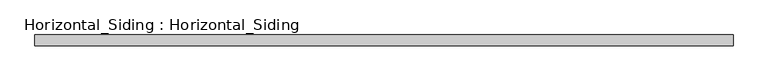
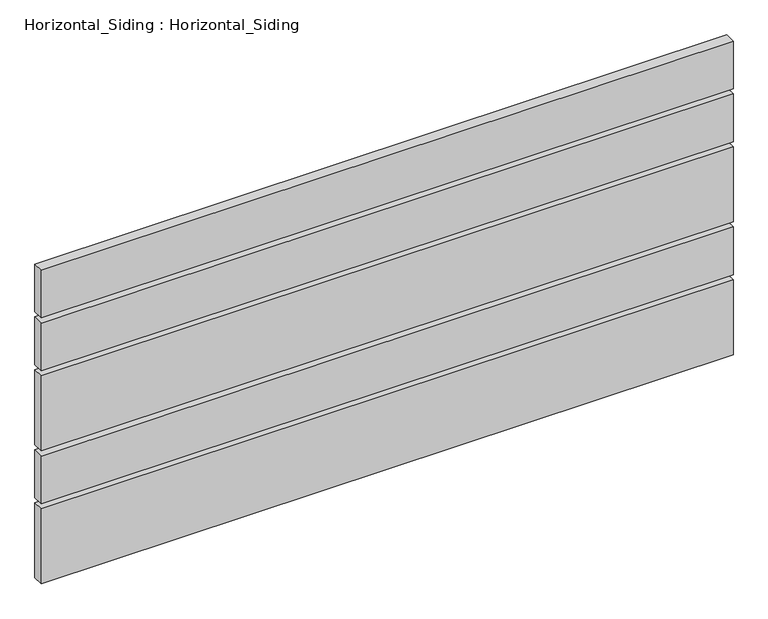
"""IFC4 building model written with IfcOpenShell, lengths in millimetres: plate geometry, Horizontal_Siding : Horizontal_Siding."""

from ifc_helpers import new_model, si_unit, frame, origin, place, context, project, spatial, polyline, outline, extrude, source, transform, mapped, element, save


def horizontal_siding_horizontal_siding_bcf56677(model_context):
    return source(origin(), model_context, "Body", "SweptSolid", [
        extrude(outline(polyline([(609.6, 19.05), (609.6, 0.0), (-609.6, 0.0), (-609.6, 19.05), (609.6, 19.05)])), frame((0.0, 0.0, 9.525), z_axis=(0.0, 0.0, 1.0), x_axis=(1.0, 0.0, 0.0)), (0.0, 0.0, 1.0), 139.7),
        extrude(outline(polyline([(609.6, 19.05), (609.6, 0.0), (-609.6, 0.0), (-609.6, 19.05), (609.6, 19.05)])), frame((0.0, 0.0, 158.75), z_axis=(0.0, 0.0, 1.0), x_axis=(1.0, 0.0, 0.0)), (0.0, 0.0, 1.0), 88.9),
        extrude(outline(polyline([(609.6, 19.05), (609.6, 0.0), (-609.6, 0.0), (-609.6, 19.05), (609.6, 19.05)])), frame((0.0, 0.0, 257.175), z_axis=(0.0, 0.0, 1.0), x_axis=(1.0, 0.0, 0.0)), (0.0, 0.0, 1.0), 139.7),
        extrude(outline(polyline([(609.6, 19.05), (609.6, 0.0), (-609.6, 0.0), (-609.6, 19.05), (609.6, 19.05)])), frame((0.0, 0.0, 406.4), z_axis=(0.0, 0.0, 1.0), x_axis=(1.0, 0.0, 0.0)), (0.0, 0.0, 1.0), 88.9),
        extrude(outline(polyline([(609.6, 19.05), (609.6, 0.0), (-609.6, 0.0), (-609.6, 19.05), (609.6, 19.05)])), frame((0.0, 0.0, 504.825), z_axis=(0.0, 0.0, 1.0), x_axis=(1.0, 0.0, 0.0)), (0.0, 0.0, 1.0), 88.9),
    ])


if __name__ == "__main__":
    model = new_model("IFC4")
    model_context = context("Model", 3, world=origin())
    ifc_project = project(units=[si_unit("LENGTHUNIT", "METRE", prefix="MILLI")], contexts=[model_context])
    site = spatial("IfcSite", under=ifc_project)
    building = spatial("IfcBuilding", under=site)
    placement = place(None, origin())
    horizontal_siding_horizontal_siding_shape = horizontal_siding_horizontal_siding_bcf56677(model_context)
    element("IfcPlate", 1, ObjectType="Horizontal_Siding : Horizontal_Siding", at=placement, inside=building, context=model_context, shape_type="MappedRepresentation", body=[
        mapped(horizontal_siding_horizontal_siding_shape, transform((0.0, 0.0, 0.0), x_axis=(1.0, 0.0, 0.0), y_axis=(0.0, 1.0, 0.0), z_axis=(0.0, 0.0, 1.0))),
    ])
    save(model, "model.ifc")

# Revit data of these elements
# Type "Horizontal_Siding : Horizontal_Siding"
#   Type Mark = "OUT"
#   Analytic Construction = "<None>"
#   extend = 0' - 2 3/4"
#   Width_2 = 0' - 3 1/2"
#   Width_1 = 0' - 5 1/2"
#   Gap = 0' - 0 3/8"
#   Plank Material = EXISTING HORZ. (1X4 & 1X6) WOOD SIDING (UNGROOVED PROFILE)
# Element 1 (IfcPlate, "Horizontal_Siding : Horizontal_Siding")
#   Materials on its faces: "EXISTING HORZ. (1X4 & 1X6) WOOD SIDING (UNGROOVED PROFILE)"
# Materials
#   "EXISTING HORZ. (1X4 & 1X6) WOOD SIDING (UNGROOVED PROFILE)": class "Wood", colour RGB 164 134 123, transparency 0, Description = "Pinus Echinata", Cost = 0
